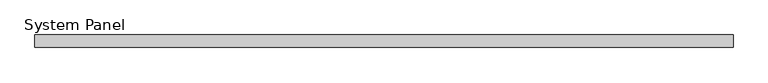
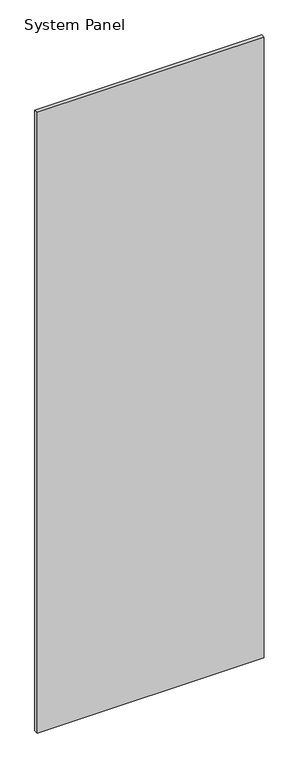
"""IFC4 building model written with IfcOpenShell, lengths in millimetres: plate geometry, System Panel : WWm-Glass-20mm-10mmOffset."""

from ifc_helpers import new_model, si_unit, origin, origin_with_axes, place, context, project, spatial, polyline, outline, extrude, source, transform, mapped, element, save


def system_panel_02ad7bca(model_context):
    return source(origin(), model_context, "Body", "SweptSolid", [
        extrude(outline(polyline([(562.5, 0.0), (-562.5, 0.0), (-562.5, 20.0), (562.5, 20.0), (562.5, 0.0)])), origin_with_axes(), (0.0, 0.0, 1.0), 3250.0),
    ])


if __name__ == "__main__":
    model = new_model("IFC4")
    model_context = context("Model", 3, world=origin())
    ifc_project = project(units=[si_unit("LENGTHUNIT", "METRE", prefix="MILLI")], contexts=[model_context])
    site = spatial("IfcSite", under=ifc_project)
    building = spatial("IfcBuilding", under=site)
    placement = place(None, origin())
    system_panel_shape = system_panel_02ad7bca(model_context)
    element("IfcPlate", 1, ObjectType="System Panel : WWm-Glass-20mm-10mmOffset", at=placement, inside=building, context=model_context, shape_type="MappedRepresentation", body=[
        mapped(system_panel_shape, transform((0.0, 0.0, 0.0), x_axis=(1.0, 0.0, 0.0), y_axis=(0.0, 1.0, 0.0), z_axis=(0.0, 0.0, 1.0))),
    ])
    save(model, "model.ifc")

# Revit data of these elements
# Type "System Panel : WWm-Glass-20mm-10mmOffset"
#   Finish = ""
# Element 1 (IfcPlate, "System Panel : WWm-Glass-20mm-10mmOffset")
#   Materials on its faces: "WW-EC-GL-Storefront"
# Materials
#   "WW-EC-GL-Storefront": class "Glass", colour RGB 236 240 239, transparency 0.85, Description = "Storefront Glass", Cost = 0
